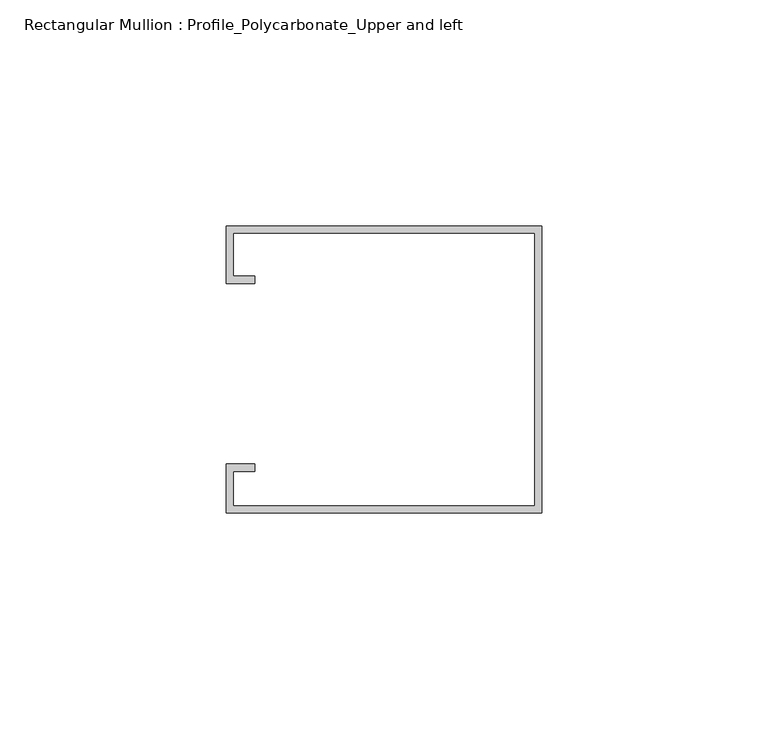
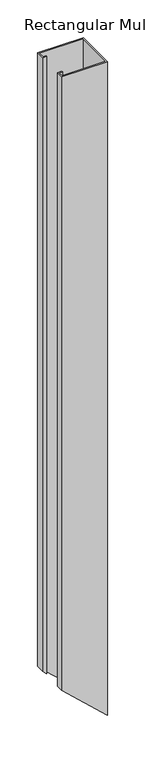
"""IFC4 building model written with IfcOpenShell, lengths in millimetres: member geometry, Rectangular Mullion : Profile_Polycarbonate_Upper and left."""

from ifc_helpers import new_model, si_unit, origin, place, context, project, spatial, faceted_brep, source, transform, mapped, element, save


def rectangular_mullion_profile_polycarbonate_upper_and_left_088f7f44(model_context):
    return source(origin(), model_context, "Body", "Brep", [
        faceted_brep([(0.0, 32.7, 0.0), (-69.85, 32.7, 0.0), (-69.85, 20.0, 0.0), (-63.5, 20.0, 0.0), (-63.5, 21.5875, 0.0), (-68.2625, 21.5875, 0.0), (-68.2625, 31.1125, 0.0), (-1.5875, 31.1125, 0.0), (-1.5875, -29.2125, 0.0), (-68.2625, -29.2125, 0.0), (-68.2625, -21.5875, 0.0), (-63.5, -21.5875, 0.0), (-63.5, -20.0, 0.0), (-69.85, -20.0, 0.0), (-69.85, -30.8, 0.0), (0.0, -30.8, 0.0), (0.0, 32.7, -1054.4076584), (-69.85, 32.7, -990.1363766), (-69.85, 20.0, -990.1363766), (-63.5, 20.0, -995.9792204), (-63.5, 21.5875, -995.9792204), (-68.2625, 21.5875, -991.5970876), (-68.2625, 31.1125, -991.5970876), (-1.5875, 31.1125, -1052.9469475), (-1.5875, -29.2125, -1052.9469475), (-68.2625, -29.2125, -991.5970876), (-68.2625, -21.5875, -991.5970876), (-63.5, -21.5875, -995.9792204), (-63.5, -20.0, -995.9792204), (-69.85, -20.0, -990.1363766), (-69.85, -30.8, -990.1363766), (0.0, -30.8, -1054.4076584)], [[[0, 1, 2, 3, 4, 5, 6, 7, 8, 9, 10, 11, 12, 13, 14, 15]], [[1, 0, 16, 17]], [[2, 1, 17, 18]], [[3, 2, 18, 19]], [[4, 3, 19, 20]], [[5, 4, 20, 21]], [[6, 5, 21, 22]], [[7, 6, 22, 23]], [[8, 7, 23, 24]], [[9, 8, 24, 25]], [[10, 9, 25, 26]], [[11, 10, 26, 27]], [[12, 11, 27, 28]], [[13, 12, 28, 29]], [[14, 13, 29, 30]], [[15, 14, 30, 31]], [[0, 15, 31, 16]], [[16, 31, 30, 29, 28, 27, 26, 25, 24, 23, 22, 21, 20, 19, 18, 17]]]),
    ])


if __name__ == "__main__":
    model = new_model("IFC4")
    model_context = context("Model", 3, world=origin())
    ifc_project = project(units=[si_unit("LENGTHUNIT", "METRE", prefix="MILLI")], contexts=[model_context])
    site = spatial("IfcSite", under=ifc_project)
    building = spatial("IfcBuilding", under=site)
    placement = place(None, origin())
    rectangular_mullion_profile_polycarbonate_upper_and_left_shape = rectangular_mullion_profile_polycarbonate_upper_and_left_088f7f44(model_context)
    element("IfcMember", 1, ObjectType="Rectangular Mullion : Profile_Polycarbonate_Upper and left", at=placement, inside=building, context=model_context, shape_type="MappedRepresentation", body=[
        mapped(rectangular_mullion_profile_polycarbonate_upper_and_left_shape, transform((0.0, 0.0, 0.0), x_axis=(1.0, 0.0, 0.0), y_axis=(0.0, 1.0, 0.0), z_axis=(0.0, 0.0, 1.0))),
    ])
    save(model, "model.ifc")

# Revit data of these elements
# Type "Rectangular Mullion : Profile_Polycarbonate_Upper and left"
#   built-in parameter 1007322 = 0.208333 (stored number, unit not read)
#   built-in parameter 1007321 = 0.00520833 (stored number, unit not read)
#   built-in parameter 1007320 = 0 (stored number, unit not read)
# Element 1 (IfcMember, "Rectangular Mullion : Profile_Polycarbonate_Upper and left")
#   Materials on its faces: "ALUMINUM PROFILE AT POLYCARBONATE PANEL"
# Materials
#   "ALUMINUM PROFILE AT POLYCARBONATE PANEL": class "Metal", colour RGB 244 244 244, transparency 0, Description = "Aluminum 6061", Cost = 0
